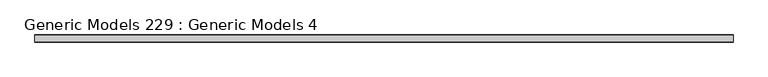
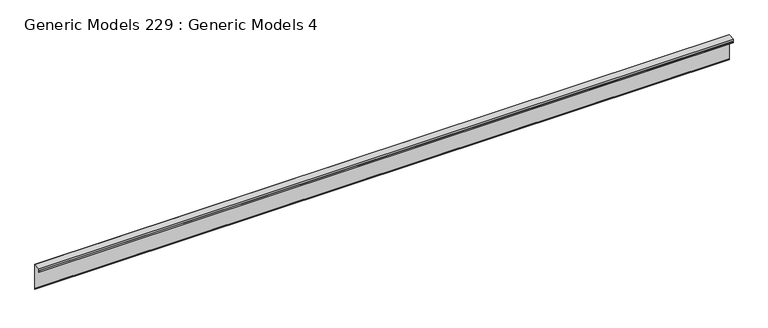
"""IFC4 building model written with IfcOpenShell, lengths in millimetres: proxy geometry, Generic Models 229 : Generic Models 4."""

from ifc_helpers import new_model, si_unit, frame, origin, place, context, project, spatial, polyline, outline, extrude, source, transform, mapped, element, save


def generic_models_229_generic_models_4_b0f16030(model_context):
    return source(origin(), model_context, "Body", "SweptSolid", [
        extrude(outline(polyline([(11781.6631007, 127013.3250789), (11781.6631007, 126974.0744351), (11780.8693507, 126974.0744351), (11780.8693507, 127013.4650384), (11783.4651647, 127020.596979), (11783.4651647, 127078.9254539), (11966.9669354, 127086.571361), (11966.9669354, 126411.2969267), (11970.2109788, 126402.3839906), (11970.2109788, 126383.3614781), (11969.4172288, 126383.3614781), (11969.4172288, 126402.2440311), (11966.1731854, 126411.1569671), (11966.1731854, 127085.7438493), (11784.2589147, 127078.1640881), (11784.2589147, 127020.4570194), (11781.6631007, 127013.3250789)])), frame((-10234.5171316, 0.0, 0.0), z_axis=(1.0, 0.0, 0.0), x_axis=(0.0, 1.0, 0.0)), (0.0, 0.0, 1.0), 18643.6),
    ])


if __name__ == "__main__":
    model = new_model("IFC4")
    model_context = context("Model", 3, world=origin())
    ifc_project = project(units=[si_unit("LENGTHUNIT", "METRE", prefix="MILLI")], contexts=[model_context])
    site = spatial("IfcSite", under=ifc_project)
    building = spatial("IfcBuilding", under=site)
    placement = place(None, origin())
    generic_models_229_generic_models_4_shape = generic_models_229_generic_models_4_b0f16030(model_context)
    element("IfcBuildingElementProxy", 1, Name="Generic Models 229 : Generic Models 4", ObjectType="Generic Models 229 : Generic Models 4", at=placement, inside=building, context=model_context, shape_type="MappedRepresentation", body=[
        mapped(generic_models_229_generic_models_4_shape, transform((0.0, 0.0, 0.0), x_axis=(1.0, 0.0, 0.0), y_axis=(0.0, 1.0, 0.0), z_axis=(0.0, 0.0, 1.0))),
    ])
    save(model, "model.ifc")

# Revit data of these elements
# Element 1 (IfcBuildingElementProxy, "Generic Models 229 : Generic Models 4")
#   Materials on its faces: "_(2) LAYERS NO. 30 ASTM D226 ASPHALT SATURATED ORGANIC FELT"
# Materials
#   "_(2) LAYERS NO. 30 ASTM D226 ASPHALT SATURATED ORGANIC FELT": class "Generic", colour RGB 67 154 161, transparency 0, Cost = 0
